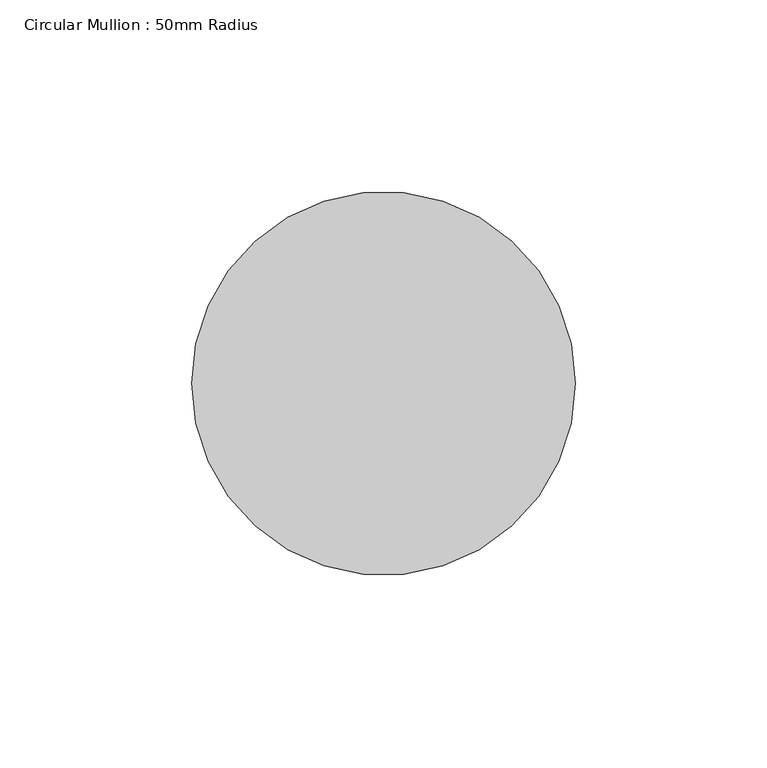
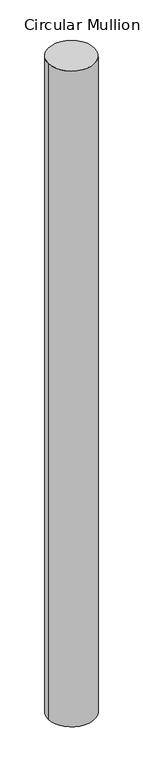
"""IFC4 building model written with IfcOpenShell, lengths in millimetres: member geometry, Circular Mullion : 50mm Radius."""

import ifcopenshell
import ifcopenshell.guid

model = None  # the IFC model being written
_history = None  # IfcOwnerHistory: only IFC2X3 demands one
_inside = {}  # id of a spatial element -> (the spatial element, [elements in it])
_under = {}  # id of a project, library or spatial element -> (it, [spatial elements below it])
_declared = {}  # id of a project -> (the project, [libraries it declares])
_typed = {}  # id of a type object -> (the type object, [elements of that type])
_made_of = {}  # id of a material, layer set ... -> (it, [elements and type objects made of it])


def new_model(schema):
    """Start an empty IFC model of exactly this schema.

    Asked for "IFC4X3", IfcOpenShell would pick the latest addendum, in which some entities
    have other attributes; the version numbers below select the first issue.
    IFC2X3 requires an IfcOwnerHistory on every rooted entity: one is made here for all.
    """
    global model, _history
    if schema == "IFC4X3":
        model = ifcopenshell.file(schema_version=(4, 3, 0, 0))
    else:
        model = ifcopenshell.file(schema=schema)
    _inside.clear()
    _under.clear()
    _declared.clear()
    _typed.clear()
    _made_of.clear()
    _history = None
    if model.schema == "IFC2X3":
        org = make("IfcOrganization", Name="unknown")
        user = make(
            "IfcPersonAndOrganization",
            ThePerson=make("IfcPerson", FamilyName="unknown"),
            TheOrganization=org,
        )
        app = make(
            "IfcApplication",
            ApplicationDeveloper=org,
            Version="unknown",
            ApplicationFullName="unknown",
            ApplicationIdentifier="unknown",
        )
        _history = make(
            "IfcOwnerHistory",
            OwningUser=user,
            OwningApplication=app,
            ChangeAction="ADDED",
            CreationDate=0,
        )
    return model


def make(cls, **values):
    """One entity of the class cls with the attributes given. An attribute that is None is left unset."""
    return model.create_entity(
        cls, **{name: value for name, value in values.items() if value is not None}
    )


def rooted(cls, **values):
    """An entity with a GlobalId (a new one), such as an element, a storey or a relation."""
    return make(cls, GlobalId=ifcopenshell.guid.new(), OwnerHistory=_history, **values)


def si_unit(unit_type, name, prefix=None):
    """IfcSIUnit, for example si_unit("LENGTHUNIT", "METRE", prefix="MILLI")."""
    return make("IfcSIUnit", UnitType=unit_type, Prefix=prefix, Name=name)


def assignment(units):
    """IfcUnitAssignment: the units of a project."""
    return None if units is None else make("IfcUnitAssignment", Units=units)


def point(xyz):
    """IfcCartesianPoint."""
    return None if xyz is None else make("IfcCartesianPoint", Coordinates=xyz)


def direction(xyz):
    """IfcDirection."""
    return None if xyz is None else make("IfcDirection", DirectionRatios=xyz)


def frame(location, z_axis=None, x_axis=None):
    """IfcAxis2Placement3D, a coordinate frame: its origin and axes. An axis left out is left unset."""
    return make(
        "IfcAxis2Placement3D",
        Location=point(location),
        Axis=direction(z_axis),
        RefDirection=direction(x_axis),
    )


def frame_2d(location, x_axis=None):
    """IfcAxis2Placement2D, a coordinate frame in the plane: its origin and x axis."""
    return make(
        "IfcAxis2Placement2D", Location=point(location), RefDirection=direction(x_axis)
    )


def origin():
    """The frame at (0, 0, 0) with its axes left unset."""
    return frame((0.0, 0.0, 0.0))


def origin_2d():
    """The frame at (0, 0) in the plane with its x axis left unset."""
    return frame_2d((0.0, 0.0))


def place(relative_to, where):
    """IfcLocalPlacement: puts the frame where relative to a parent placement (None: the world)."""
    return make(
        "IfcLocalPlacement", PlacementRelTo=relative_to, RelativePlacement=where
    )


def context(
    kind, dimensions, precision=None, world=None, true_north=None, identifier=None
):
    """IfcGeometricRepresentationContext, for example the 3D "Model" context."""
    return make(
        "IfcGeometricRepresentationContext",
        ContextIdentifier=identifier,
        ContextType=kind,
        CoordinateSpaceDimension=dimensions,
        Precision=precision,
        WorldCoordinateSystem=world,
        TrueNorth=true_north,
    )


def project(units=None, contexts=None):
    """IfcProject with its units and contexts."""
    return rooted(
        "IfcProject",
        Name="project",
        RepresentationContexts=contexts,
        UnitsInContext=assignment(units),
    )


def spatial(cls, under=None, at=None, **own):
    """A site, building, storey or space (cls), placed at a placement, below another one or the project."""
    s = rooted(cls, ObjectPlacement=at, **own)
    if under is not None:
        _under.setdefault(under.id(), (under, []))[1].append(s)
    return s


def circle_curve(where, radius):
    """IfcCircle in the frame where."""
    return make("IfcCircle", Position=where, Radius=radius)


def trimmed(basis, trim1, trim2, sense, master):
    """IfcTrimmedCurve: the piece of a basis curve between two trims."""
    return make(
        "IfcTrimmedCurve",
        BasisCurve=basis,
        Trim1=trim1,
        Trim2=trim2,
        SenseAgreement=sense,
        MasterRepresentation=master,
    )


def segment(curve, same_sense, transition):
    """IfcCompositeCurveSegment."""
    return make(
        "IfcCompositeCurveSegment",
        Transition=transition,
        SameSense=same_sense,
        ParentCurve=curve,
    )


def composite_curve(segments, self_intersect=None):
    """IfcCompositeCurve: segments joined end to end."""
    return make("IfcCompositeCurve", Segments=segments, SelfIntersect=self_intersect)


def outline(outer, holes=None, kind="AREA"):
    """IfcArbitraryClosedProfileDef: a profile drawn as a closed curve; with holes, ...WithVoids."""
    if holes is None:
        return make("IfcArbitraryClosedProfileDef", ProfileType=kind, OuterCurve=outer)
    return make(
        "IfcArbitraryProfileDefWithVoids",
        ProfileType=kind,
        OuterCurve=outer,
        InnerCurves=holes,
    )


def extrude(swept, where, along, depth):
    """IfcExtrudedAreaSolid: the profile swept, set in the frame where, extruded along a direction by depth."""
    return make(
        "IfcExtrudedAreaSolid",
        SweptArea=swept,
        Position=where,
        ExtrudedDirection=direction(along),
        Depth=depth,
    )


def shape(context_of_items, identifier, shape_type, items):
    """IfcShapeRepresentation: the items that make up one representation, for example the "Body"."""
    return make(
        "IfcShapeRepresentation",
        ContextOfItems=context_of_items,
        RepresentationIdentifier=identifier,
        RepresentationType=shape_type,
        Items=items,
    )


def source(mapping_origin, context_of_items, identifier, shape_type, items):
    """IfcRepresentationMap: a shape defined once, which mapped items show again and again."""
    return make(
        "IfcRepresentationMap",
        MappingOrigin=mapping_origin,
        MappedRepresentation=shape(context_of_items, identifier, shape_type, items),
    )


def transform(
    local_origin,
    x_axis=None,
    y_axis=None,
    z_axis=None,
    scale=None,
    scale2=None,
    scale3=None,
    uniform=True,
):
    """IfcCartesianTransformationOperator3D, or its non-uniform kind. x_axis, y_axis, z_axis: its Axis1, 2, 3."""
    if uniform:
        return make(
            "IfcCartesianTransformationOperator3D",
            Axis1=direction(x_axis),
            Axis2=direction(y_axis),
            LocalOrigin=point(local_origin),
            Scale=scale,
            Axis3=direction(z_axis),
        )
    return make(
        "IfcCartesianTransformationOperator3DnonUniform",
        Axis1=direction(x_axis),
        Axis2=direction(y_axis),
        LocalOrigin=point(local_origin),
        Scale=scale,
        Axis3=direction(z_axis),
        Scale2=scale2,
        Scale3=scale3,
    )


def mapped(mapping_source, mapping_target):
    """IfcMappedItem: shows the shape of a source again, moved by a transform."""
    return make(
        "IfcMappedItem", MappingSource=mapping_source, MappingTarget=mapping_target
    )


def made_of(thing, what):
    """Note that an element or type object is made of a material, layer set ...; save() writes the relation."""
    if what is not None:
        _made_of.setdefault(what.id(), (what, []))[1].append(thing)
    return thing


def element(
    cls,
    number,
    at=None,
    inside=None,
    cuts=None,
    type_object=None,
    material=None,
    context=None,
    identifier="Body",
    shape_type=None,
    held_by="IfcProductDefinitionShape",
    body=None,
    shapes=None,
    **own,
):
    """One element of the class cls, such as IfcWall. Its Tag is "e" and its number.

    at: its placement. inside: the storey or other place that contains it. cuts: it is an
    opening in that element (IfcRelVoidsElement). A single representation is given by context,
    identifier, shape_type and body (its items); several are given by shapes. held_by: the class
    of the entity that holds the representations. save() writes the other relations.
    """
    e = rooted(cls, Tag="e%d" % number, ObjectPlacement=at, **own)
    if body is not None:
        shapes = [shape(context, identifier, shape_type, body)]
    if shapes is not None:
        e.Representation = make(held_by, Representations=shapes)
    if inside is not None:
        _inside.setdefault(inside.id(), (inside, []))[1].append(e)
    if cuts is not None:
        rooted(
            "IfcRelVoidsElement", RelatingBuildingElement=cuts, RelatedOpeningElement=e
        )
    if type_object is not None:
        _typed.setdefault(type_object.id(), (type_object, []))[1].append(e)
    return made_of(e, material)


def aggregate(whole, parts):
    """IfcRelAggregates: a whole, such as a stair, and the parts it consists of."""
    return rooted("IfcRelAggregates", RelatingObject=whole, RelatedObjects=parts)


def save(model, path):
    """Write the relations noted so far, then the file.

    IfcRelAggregates (storeys below a building ...), IfcRelContainedInSpatialStructure (elements
    in a storey), IfcRelDefinesByType, IfcRelAssociatesMaterial and IfcRelDeclares: one each for
    every whole, place, type object, material and project.
    """
    for whole, parts in _under.values():
        aggregate(whole, parts)
    for where, things in _inside.values():
        rooted(
            "IfcRelContainedInSpatialStructure",
            RelatedElements=things,
            RelatingStructure=where,
        )
    for kind, things in _typed.values():
        rooted("IfcRelDefinesByType", RelatedObjects=things, RelatingType=kind)
    for what, things in _made_of.values():
        rooted("IfcRelAssociatesMaterial", RelatedObjects=things, RelatingMaterial=what)
    for by, libraries in _declared.values():
        rooted("IfcRelDeclares", RelatingContext=by, RelatedDefinitions=libraries)
    model.write(path)


def circular_mullion_50mm_radius_0cb45251(model_context):
    return source(origin(), model_context, "Body", "SweptSolid", [
        extrude(outline(composite_curve([segment(trimmed(circle_curve(origin_2d(), 50.0), [point((50.0, 0.0))], [point((-50.0, 0.0))], False, "CARTESIAN"), True, "CONTINUOUS"), segment(trimmed(circle_curve(origin_2d(), 50.0), [point((-50.0, 0.0))], [point((50.0, 0.0))], False, "CARTESIAN"), True, "CONTINUOUS")], self_intersect=False)), frame((0.0, 0.0, -1500.9280484), z_axis=(0.0, 0.0, 1.0), x_axis=(1.0, 0.0, 0.0)), (0.0, 0.0, 1.0), 1500.9280484),
    ])


if __name__ == "__main__":
    model = new_model("IFC4")
    model_context = context("Model", 3, world=origin())
    ifc_project = project(units=[si_unit("LENGTHUNIT", "METRE", prefix="MILLI")], contexts=[model_context])
    site = spatial("IfcSite", under=ifc_project)
    building = spatial("IfcBuilding", under=site)
    placement = place(None, origin())
    circular_mullion_50mm_radius_shape = circular_mullion_50mm_radius_0cb45251(model_context)
    element("IfcMember", 1, ObjectType="Circular Mullion : 50mm Radius", at=placement, inside=building, context=model_context, shape_type="MappedRepresentation", body=[
        mapped(circular_mullion_50mm_radius_shape, transform((0.0, 0.0, 0.0), x_axis=(1.0, 0.0, 0.0), y_axis=(0.0, 1.0, 0.0), z_axis=(0.0, 0.0, 1.0))),
    ])
    save(model, "model.ifc")

# Revit data of these elements
# Type "Circular Mullion : 50mm Radius"
#   built-in parameter 1007350 = 0.164042 (stored number, unit not read)
# Element 1 (IfcMember, "Circular Mullion : 50mm Radius")
#   Materials on its faces: "Aluminium"
# Materials
#   "Aluminium": class "Metal", colour RGB 247 247 247, transparency 0, Description = "Aluminium 6061", Cost = 0
